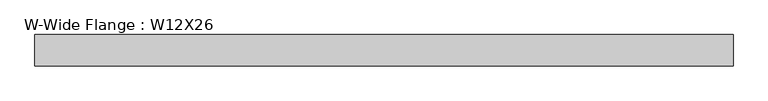
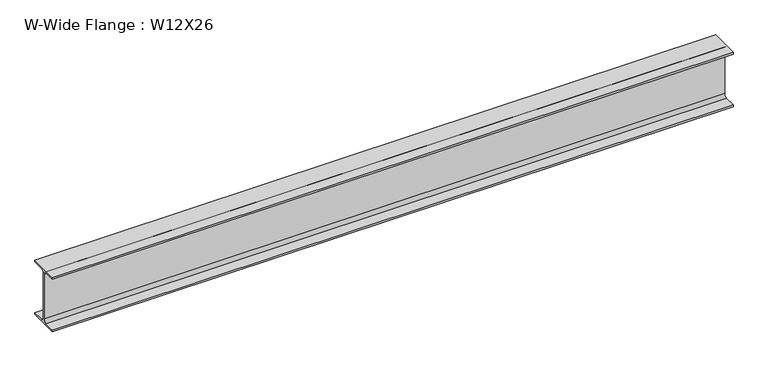
"""IFC4 building model written with IfcOpenShell, lengths in millimetres: beam geometry, W-Wide Flange : W12X26."""

from ifc_helpers import new_model, si_unit, point, frame, frame_2d, origin, place, context, project, spatial, polyline, circle_curve, trimmed, segment, composite_curve, outline, extrude, source, transform, mapped, element, save


def w_wide_flange_w12x26_a2670070(model_context):
    return source(origin(), model_context, "Body", "SweptSolid", [
        extrude(outline(composite_curve([segment(polyline([(82.423, -145.288), (82.423, -154.94), (-82.423, -154.94), (-82.423, -145.288), (-20.2565, -145.288)]), True, "CONTINUOUS"), segment(trimmed(circle_curve(frame_2d((-20.2565, -127.9525)), 17.3355), [point((-20.2565, -145.288))], [point((-2.921, -127.9525))], True, "CARTESIAN"), True, "CONTINUOUS"), segment(polyline([(-2.921, -127.9525), (-2.921, 127.9525)]), True, "CONTINUOUS"), segment(trimmed(circle_curve(frame_2d((-20.2565, 127.9525)), 17.3355), [point((-2.921, 127.9525))], [point((-20.2565, 145.288))], True, "CARTESIAN"), True, "CONTINUOUS"), segment(polyline([(-20.2565, 145.288), (-82.423, 145.288), (-82.423, 154.94), (82.423, 154.94), (82.423, 145.288), (20.2565, 145.288)]), True, "CONTINUOUS"), segment(trimmed(circle_curve(frame_2d((20.2565, 127.9525)), 17.3355), [point((20.2565, 145.288))], [point((2.921, 127.9525))], True, "CARTESIAN"), True, "CONTINUOUS"), segment(polyline([(2.921, 127.9525), (2.921, -127.9525)]), True, "CONTINUOUS"), segment(trimmed(circle_curve(frame_2d((20.2565, -127.9525)), 17.3355), [point((2.921, -127.9525))], [point((20.2565, -145.288))], True, "CARTESIAN"), True, "CONTINUOUS"), segment(polyline([(20.2565, -145.288), (82.423, -145.288)]), True, "CONTINUOUS")], self_intersect=False)), frame((-1787.5760943, 0.0, 0.0), z_axis=(1.0, 0.0, 0.0), x_axis=(0.0, 1.0, 0.0)), (0.0, 0.0, 1.0), 3683.0),
    ])


if __name__ == "__main__":
    model = new_model("IFC4")
    model_context = context("Model", 3, world=origin())
    ifc_project = project(units=[si_unit("LENGTHUNIT", "METRE", prefix="MILLI")], contexts=[model_context])
    site = spatial("IfcSite", under=ifc_project)
    building = spatial("IfcBuilding", under=site)
    placement = place(None, origin())
    w_wide_flange_w12x26_shape = w_wide_flange_w12x26_a2670070(model_context)
    element("IfcBeam", 1, ObjectType="W-Wide Flange : W12X26", at=placement, inside=building, context=model_context, shape_type="MappedRepresentation", body=[
        mapped(w_wide_flange_w12x26_shape, transform((0.0, 0.0, 0.0), x_axis=(1.0, 0.0, 0.0), y_axis=(0.0, 1.0, 0.0), z_axis=(0.0, 0.0, 1.0))),
    ])
    save(model, "model.ifc")

# Revit data of these elements
# Type "W-Wide Flange : W12X26"
#   Assembly Code = "B10"
#   W = 26
#   Length [instance default] = 5' - 0"
#   bf = 0' - 6.49"
#   d = 1' - 0.2"
#   k = 0' - 1 1/16"
#   k2 = 0' - 0.6825"
#   tf = 0' - 0.38"
#   tw = 0' - 0.23"
#   A = 0.053125 SF
#   Structural Material [instance default] = Steel ASTM A992
# Element 1 (IfcBeam, "W-Wide Flange : W12X26")
#   Materials on its faces: "Steel ASTM A992"
# Materials
#   "Steel ASTM A992": class "Metal", colour RGB 199 199 199, transparency 0, Description = "Structural steel 50ksi", Cost = 0
